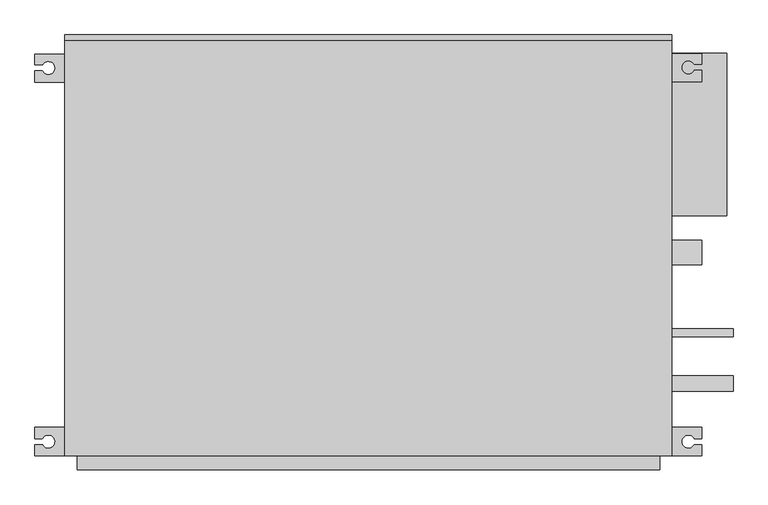
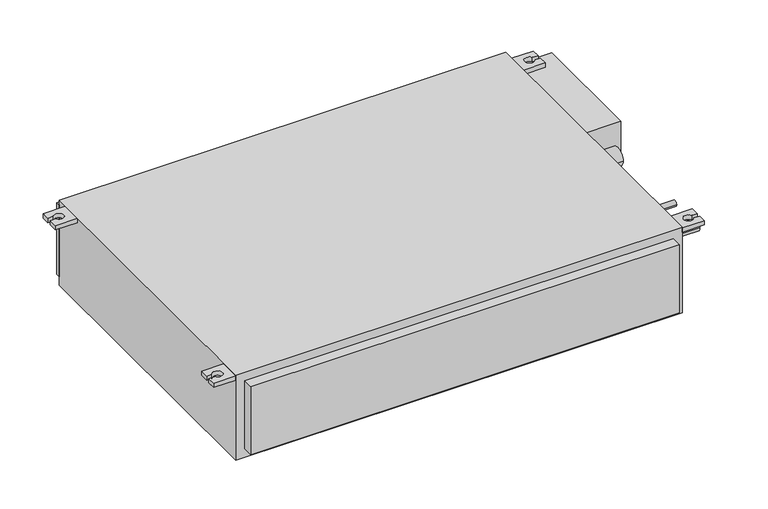
"""IFC4 building model written with IfcOpenShell, lengths in millimetres: proxy geometry, PEFY-P-NMSU-E_Low_Profile_Ducted : PEFY-P15NMSU-E."""

from ifc_helpers import new_model, si_unit, point, frame, frame_2d, origin, origin_with_axes, place, context, project, spatial, polyline, circle_curve, trimmed, segment, composite_curve, outline, extrude, source, transform, mapped, element, save


def mechanical_equipment_be926906(model_context):
    return source(origin(), model_context, "Body", "SweptSolid", [
        extrude(outline(composite_curve([segment(polyline([(-544.3, 282.0), (-544.3, 300.9759165), (-532.1454311, 300.9759165)]), True, "CONTINUOUS"), segment(trimmed(circle_curve(frame_2d((-522.2863556, 305.4254582)), 10.8166442), [point((-532.1454311, 300.9759165))], [point((-531.8387803, 310.5))], True, "CARTESIAN"), True, "CONTINUOUS"), segment(polyline([(-531.8387803, 310.5), (-544.3, 310.5), (-544.3, 328.0), (-495.3, 328.0), (-495.3, 282.0), (-544.3, 282.0)]), True, "CONTINUOUS")], self_intersect=False)), frame((0.0, 0.0, 188.55), z_axis=(0.0, 0.0, 1.0), x_axis=(1.0, 0.0, 0.0)), (0.0, 0.0, 1.0), 10.0),
        extrude(outline(composite_curve([segment(polyline([(-544.3, -281.0), (-495.3, -281.0), (-495.3, -327.0), (-544.3, -327.0), (-544.3, -309.5), (-531.8387803, -309.5)]), True, "CONTINUOUS"), segment(trimmed(circle_curve(frame_2d((-522.2863556, -304.4254582)), 10.8166442), [point((-531.8387803, -309.5))], [point((-532.1454311, -299.9759165))], True, "CARTESIAN"), True, "CONTINUOUS"), segment(polyline([(-532.1454311, -299.9759165), (-544.3, -299.9759165), (-544.3, -281.0)]), True, "CONTINUOUS")], self_intersect=False)), frame((0.0, 0.0, 188.55), z_axis=(0.0, 0.0, 1.0), x_axis=(1.0, 0.0, 0.0)), (0.0, 0.0, 1.0), 10.0),
        extrude(outline(composite_curve([segment(polyline([(544.3, 282.9429009), (495.3, 282.9429009), (495.3, 328.9429009), (544.3, 328.9429009), (544.3, 311.4429009), (531.8387803, 311.4429009)]), True, "CONTINUOUS"), segment(trimmed(circle_curve(frame_2d((522.2863556, 306.3683591)), 10.8166442), [point((531.8387803, 311.4429009))], [point((532.1454311, 301.9188174))], True, "CARTESIAN"), True, "CONTINUOUS"), segment(polyline([(532.1454311, 301.9188174), (544.3, 301.9188174), (544.3, 282.9429009)]), True, "CONTINUOUS")], self_intersect=False)), frame((0.0, 0.0, 188.55), z_axis=(0.0, 0.0, 1.0), x_axis=(1.0, 0.0, 0.0)), (0.0, 0.0, 1.0), 10.0),
        extrude(outline(composite_curve([segment(polyline([(544.3, -281.0), (544.3, -299.9759165), (532.1454311, -299.9759165)]), True, "CONTINUOUS"), segment(trimmed(circle_curve(frame_2d((522.2863556, -304.4254582)), 10.8166442), [point((532.1454311, -299.9759165))], [point((531.8387803, -309.5))], True, "CARTESIAN"), True, "CONTINUOUS"), segment(polyline([(531.8387803, -309.5), (544.3, -309.5), (544.3, -327.0), (495.3, -327.0), (495.3, -281.0), (544.3, -281.0)]), True, "CONTINUOUS")], self_intersect=False)), frame((0.0, 0.0, 188.55), z_axis=(0.0, 0.0, 1.0), x_axis=(1.0, 0.0, 0.0)), (0.0, 0.0, 1.0), 10.0),
        extrude(outline(polyline([(495.3, 350.04375), (-495.3, 350.04375), (-495.3, 359.5477547), (495.3, 359.5477547), (495.3, 350.04375)])), frame((0.0, 0.0, 20.0), z_axis=(0.0, 0.0, 1.0), x_axis=(1.0, 0.0, 0.0)), (0.0, 0.0, 1.0), 168.55),
        extrude(outline(composite_curve([segment(trimmed(circle_curve(frame_2d((4.0570991, 59.8)), 20.0421875), [point((-15.9850884, 59.8))], [point((24.0992866, 59.8))], False, "CARTESIAN"), True, "CONTINUOUS"), segment(trimmed(circle_curve(frame_2d((4.0570991, 59.8)), 20.0421875), [point((24.0992866, 59.8))], [point((-15.9850884, 59.8))], False, "CARTESIAN"), True, "CONTINUOUS")], self_intersect=False)), frame((495.3, 0.0, 0.0), z_axis=(1.0, 0.0, 0.0), x_axis=(0.0, 1.0, 0.0)), (0.0, 0.0, 1.0), 26.9863556),
        extrude(outline(composite_curve([segment(trimmed(circle_curve(frame_2d((4.0570991, 149.6)), 20.0421875), [point((-15.9850884, 149.6))], [point((24.0992866, 149.6))], False, "CARTESIAN"), True, "CONTINUOUS"), segment(trimmed(circle_curve(frame_2d((4.0570991, 149.6)), 20.0421875), [point((24.0992866, 149.6))], [point((-15.9850884, 149.6))], False, "CARTESIAN"), True, "CONTINUOUS")], self_intersect=False)), frame((495.3, 0.0, 0.0), z_axis=(1.0, 0.0, 0.0), x_axis=(0.0, 1.0, 0.0)), (0.0, 0.0, 1.0), 49.0),
        extrude(outline(composite_curve([segment(trimmed(circle_curve(frame_2d((-126.5596979, 100.0)), 6.4492188), [point((-133.0089166, 100.0))], [point((-120.1104791, 100.0))], False, "CARTESIAN"), True, "CONTINUOUS"), segment(trimmed(circle_curve(frame_2d((-126.5596979, 100.0)), 6.4492188), [point((-120.1104791, 100.0))], [point((-133.0089166, 100.0))], False, "CARTESIAN"), True, "CONTINUOUS")], self_intersect=False)), frame((495.3, 0.0, 0.0), z_axis=(1.0, 0.0, 0.0), x_axis=(0.0, 1.0, 0.0)), (0.0, 0.0, 1.0), 100.0),
        extrude(outline(composite_curve([segment(trimmed(circle_curve(frame_2d((-209.7540575, 100.0)), 12.7), [point((-222.4540575, 100.0))], [point((-197.0540575, 100.0))], False, "CARTESIAN"), True, "CONTINUOUS"), segment(trimmed(circle_curve(frame_2d((-209.7540575, 100.0)), 12.7), [point((-197.0540575, 100.0))], [point((-222.4540575, 100.0))], False, "CARTESIAN"), True, "CONTINUOUS")], self_intersect=False)), frame((495.3, 0.0, 0.0), z_axis=(1.0, 0.0, 0.0), x_axis=(0.0, 1.0, 0.0)), (0.0, 0.0, 1.0), 100.0),
        extrude(outline(polyline([(585.3, 330.0), (585.3, 64.0570991), (495.3, 64.0570991), (495.3, 330.0), (585.3, 330.0)])), frame((0.0, 0.0, 20.0), z_axis=(0.0, 0.0, 1.0), x_axis=(1.0, 0.0, 0.0)), (0.0, 0.0, 1.0), 159.8),
        extrude(outline(polyline([(475.3, -350.04375), (-475.3, -350.04375), (-475.3, -327.0), (475.3, -327.0), (475.3, -350.04375)])), frame((0.0, 0.0, 19.9585938), z_axis=(0.0, 0.0, 1.0), x_axis=(1.0, 0.0, 0.0)), (0.0, 0.0, 1.0), 159.8414063),
        extrude(outline(polyline([(-495.3, -327.0), (-495.3, 350.04375), (495.3, 350.04375), (495.3, -327.0), (-495.3, -327.0)])), origin_with_axes(), (0.0, 0.0, 1.0), 200.0),
    ])


if __name__ == "__main__":
    model = new_model("IFC4")
    model_context = context("Model", 3, world=origin())
    ifc_project = project(units=[si_unit("LENGTHUNIT", "METRE", prefix="MILLI")], contexts=[model_context])
    site = spatial("IfcSite", under=ifc_project)
    building = spatial("IfcBuilding", under=site)
    placement = place(None, origin())
    mechanical_equipment_shape = mechanical_equipment_be926906(model_context)
    element("IfcBuildingElementProxy", 1, Name="PEFY-P-NMSU-E_Low_Profile_Ducted : PEFY-P15NMSU-E", ObjectType="PEFY-P-NMSU-E_Low_Profile_Ducted : PEFY-P15NMSU-E", at=placement, inside=building, context=model_context, shape_type="MappedRepresentation", body=[
        mapped(mechanical_equipment_shape, transform((0.0, 0.0, 0.0), x_axis=(1.0, 0.0, 0.0), y_axis=(0.0, 1.0, 0.0), z_axis=(0.0, 0.0, 1.0))),
    ])
    save(model, "model.ifc")

# Revit data of these elements
# Type "PEFY-P-NMSU-E_Low_Profile_Ducted : PEFY-P15NMSU-E"
#   Subcategory = "HVAC"
#   Standard Air Filter = "Polypropylene Honeycomb"
#   Specification URL = "http://www.mrslim.com/customerCare/resources.asp"
#   Sound Pressure Levels (dB(A)) = "28-30-33"
#   SmartBIM Object Created By = "Reed Construction Data"
#   Refirigerant Pipe diameter (Liquid) = "1/4\""
#   Refirigerant Pipe diameter (Gas) = "1/2\""
#   Power Source = "208/230, 1, 60"
#   Power Consumption Heating = "0.05 kW"
#   Power Consumption Cooling = "0.07 kW"
#   Unit Weight (LBS) = "54"
#   Model = "PEFY-P15NMSU-E"
#   Manufacturer URL = "http://www.mrslim.com/customerCare/resources.asp"
#   Manufacturer = "Mitsubishi Electric"
#   Installation URL = "http://www.mrslim.com/customerCare/resources.asp"
#   Fan Motor Type = "DC Motor"
#   Fan Motor Output = "0.096 kW"
#   MCA = "1.20/1.33"
#   MOCP = "15 A"
#   E.S.P (In. W.G.) = ".02-.20"
#   Drainpipe Dimension = "1-1/4"
#   Description = "Ceiling Concealed Ducted Low Profile"
#   Condensate Lift Mechanism = "21-11/16\" "
#   Coil Type = "Cross Fin"
#   Heating Capacity (BTU) = "17000"
#   Fan Type x Quantity = "Sirocco Fan x 2"
#   Current Heating = "0.45 A"
#   Current Cooling = "0.55 A"
#   Cooling Capacity (BTU) = "15000"
#   Fan capacity (CFM) = "282-335-388 "
#   Assembly Code = "D3050200"
#   95 CSI = "15760"
#   04 CSI = "23 82 19 "
#   Width = 3' - 3"
#   Voltage = 0 V
#   Unit Supply Airflow [instance default] = 0 CFM
#   Unit Return Airflow [instance default] = 0 CFM
#   SmartBIM Object Version = 3
#   Height = 0' - 7.87402"
#   Drain Pipe Radius = 0' - 0 101/128"
#   Depth = 2' - 3 9/16"
#   Default Elevation = 4' - 0"
#   C = 3' - 6.85827"
#   Brazing Connection Radius (Liquid) = 0' - 0 65/256"
#   Brazing Connection Radius (Gas) = 0' - 0 1/2"
#   Suspension Bolt Pitch = 3' - 5.04724"
#   Apparent Load = 0 VA
#   Air Outlet Width = 3' - 1.4252"
#   Air Inlet Width = 3' - 3"
#   Air Outlet Height = 0' - 6 75/256"
#   Air Inlet Height = 0' - 6.65354"
#   Number of Poles = 1
#   Load Classification = Other
#   External Finish = Galvanized Steel Sheet
#   Air Outlet Unit Material = Metal Grill
#   Air Inlet Unit Material = Grill
#   URL = ""
# Element 1 (IfcBuildingElementProxy, "PEFY-P-NMSU-E_Low_Profile_Ducted : PEFY-P15NMSU-E")
#   Unit Supply Airflow = 300 CFM
#   Unit Return Airflow = 400 CFM
#   Materials on its faces: "Galvanized Steel Sheet", "Grill", "Metal Grill"
# Materials
#   "Galvanized Steel Sheet": class "Metal", colour RGB 189 187 185, transparency 0
#   "Metal Grill": class "Metal", colour RGB 10 10 10, transparency 0
#   "Grill": class "Plastic", colour RGB 5 5 5, transparency 0
